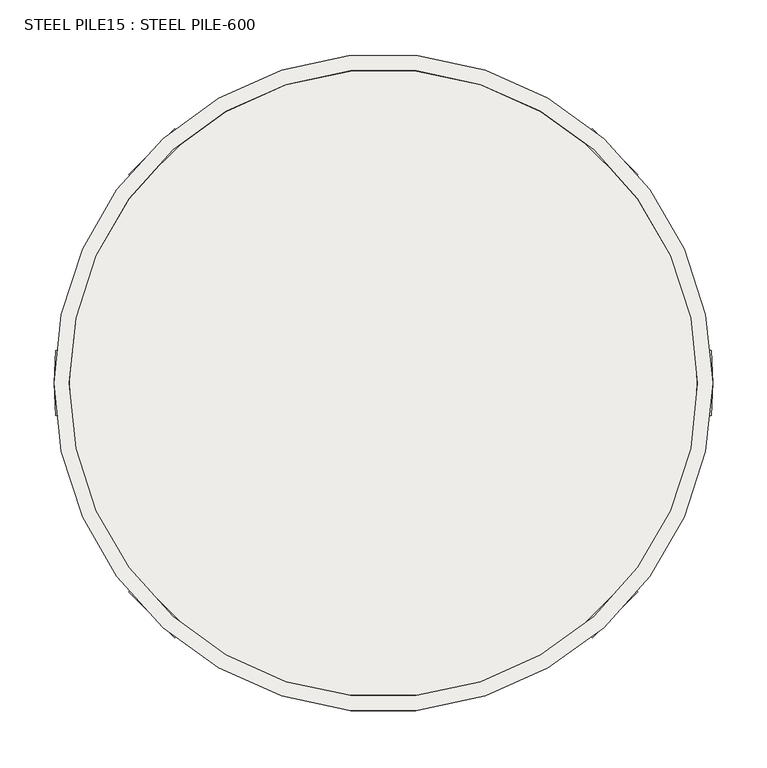
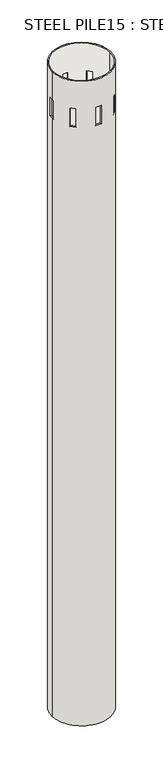
"""IFC4 building model written with IfcOpenShell, lengths in millimetres: slab geometry, STEEL PILE15 : STEEL PILE-600."""

from ifc_helpers import new_model, si_unit, point, frame, frame_2d, origin, place, context, project, spatial, polyline, circle_curve, trimmed, segment, composite_curve, outline, extrude, source, transform, mapped, element, save
from ifc_brep_helpers import plane_surface, cylinder_surface, revolved_surface, advanced_brep


def steel_pile15_steel_pile_600_f495fe2f(model_context):
    return source(origin(), model_context, "Body", "SolidModel", [
        advanced_brep(
        [(7615.5, 66679.5208589, -7500.0), (8224.5, 66679.5208589, -7500.0), (7629.5, 66679.5208589, -7500.0), (8210.5, 66679.5208589, -7500.0), (7615.5, 66679.5208589, -500.0), (8224.5, 66679.5208589, -500.0), (7629.5, 66679.5208589, -500.0), (8210.5, 66679.5208589, -500.0), (8224.5, 66679.5208589, -1000.0), (8223.0185638, 66649.5208589, -1000.0), (8223.0185638, 66649.5208589, -800.0), (8224.5, 66679.5208589, -800.0), (7615.5, 66679.5208589, -800.0), (7616.9814362, 66649.5208589, -800.0), (7616.9814362, 66649.5208589, -1000.0), (7615.5, 66679.5208589, -1000.0), (8155.4796847, 66486.467581, -1000.0), (8113.0532778, 66444.0411742, -1000.0), (8113.0532778, 66444.0411742, -800.0), (8155.4796847, 66486.467581, -800.0), (7950.0, 66376.5022951, -1000.0), (7890.0, 66376.5022951, -1000.0), (7890.0, 66376.5022951, -800.0), (7950.0, 66376.5022951, -800.0), (7726.9467222, 66444.0411742, -1000.0), (7684.5203153, 66486.467581, -1000.0), (7684.5203153, 66486.467581, -800.0), (7726.9467222, 66444.0411742, -800.0), (7616.9814362, 66709.5208589, -1000.0), (7616.9814362, 66709.5208589, -800.0), (8223.0185638, 66709.5208589, -800.0), (8223.0185638, 66709.5208589, -1000.0), (7684.5203153, 66872.5741367, -1000.0), (7726.9467222, 66915.0005436, -1000.0), (7726.9467222, 66915.0005436, -800.0), (7684.5203153, 66872.5741367, -800.0), (7890.0, 66982.5394227, -1000.0), (7950.0, 66982.5394227, -1000.0), (7950.0, 66982.5394227, -800.0), (7890.0, 66982.5394227, -800.0), (8113.0532778, 66915.0005436, -1000.0), (8155.4796847, 66872.5741367, -1000.0), (8155.4796847, 66872.5741367, -800.0), (8113.0532778, 66915.0005436, -800.0), (8210.5, 66679.5208589, -1000.0), (8208.9467944, 66709.5208589, -1000.0), (8208.9467944, 66709.5208589, -800.0), (8210.5, 66679.5208589, -800.0), (7629.5, 66679.5208589, -800.0), (7631.0532056, 66709.5208589, -800.0), (7631.0532056, 66709.5208589, -1000.0), (7629.5, 66679.5208589, -1000.0), (8145.5294412, 66862.6238932, -1000.0), (8103.1030343, 66905.0503001, -1000.0), (8103.1030343, 66905.0503001, -800.0), (8145.5294412, 66862.6238932, -800.0), (7950.0, 66968.4676533, -1000.0), (7890.0, 66968.4676533, -1000.0), (7890.0, 66968.4676533, -800.0), (7950.0, 66968.4676533, -800.0), (7736.8969657, 66905.0503001, -1000.0), (7694.4705588, 66862.6238932, -1000.0), (7694.4705588, 66862.6238932, -800.0), (7736.8969657, 66905.0503001, -800.0), (7631.0532056, 66649.5208589, -1000.0), (7631.0532056, 66649.5208589, -800.0), (8208.9467944, 66649.5208589, -800.0), (8208.9467944, 66649.5208589, -1000.0), (7694.4705588, 66496.4178246, -1000.0), (7736.8969657, 66453.9914177, -1000.0), (7736.8969657, 66453.9914177, -800.0), (7694.4705588, 66496.4178246, -800.0), (7890.0, 66390.5740645, -1000.0), (7950.0, 66390.5740645, -1000.0), (7950.0, 66390.5740645, -800.0), (7890.0, 66390.5740645, -800.0), (8103.1030343, 66453.9914177, -1000.0), (8145.5294412, 66496.4178246, -1000.0), (8145.5294412, 66496.4178246, -800.0), (8103.1030343, 66453.9914177, -800.0)],
        [
            (0, 1, circle_curve(frame((7920.0, 66679.5208589, -7500.0), z_axis=(0.0, 0.0, -1.0), x_axis=(1.0, 0.0, 0.0)), 304.5)),
            (1, 0, circle_curve(frame((7920.0, 66679.5208589, -7500.0), z_axis=(0.0, 0.0, -1.0), x_axis=(1.0, 0.0, 0.0)), 304.5)),
            (2, 3, circle_curve(frame((7920.0, 66679.5208589, -7500.0), z_axis=(0.0, 0.0, 1.0), x_axis=(1.0, 0.0, 0.0)), 290.5)),
            (3, 2, circle_curve(frame((7920.0, 66679.5208589, -7500.0), z_axis=(0.0, 0.0, 1.0), x_axis=(1.0, 0.0, 0.0)), 290.5)),
            (4, 5, circle_curve(frame((7920.0, 66679.5208589, -500.0), z_axis=(0.0, 0.0, 1.0), x_axis=(1.0, 0.0, 0.0)), 304.5)),
            (5, 4, circle_curve(frame((7920.0, 66679.5208589, -500.0), z_axis=(0.0, 0.0, 1.0), x_axis=(1.0, 0.0, 0.0)), 304.5)),
            (6, 7, circle_curve(frame((7920.0, 66679.5208589, -500.0), z_axis=(0.0, 0.0, -1.0), x_axis=(1.0, 0.0, 0.0)), 290.5)),
            (7, 6, circle_curve(frame((7920.0, 66679.5208589, -500.0), z_axis=(0.0, 0.0, -1.0), x_axis=(1.0, 0.0, 0.0)), 290.5)),
            (1, 8),
            (8, 9, circle_curve(frame((7920.0, 66679.5208589, -1000.0), z_axis=(0.0, 0.0, -1.0), x_axis=(1.0, 0.0, 0.0)), 304.5)),
            (9, 10),
            (10, 11, circle_curve(frame((7920.0, 66679.5208589, -800.0), z_axis=(0.0, 0.0, 1.0), x_axis=(1.0, 0.0, 0.0)), 304.5)),
            (11, 5),
            (4, 12),
            (12, 13, circle_curve(frame((7920.0, 66679.5208589, -800.0), z_axis=(0.0, 0.0, 1.0), x_axis=(1.0, 0.0, 0.0)), 304.5)),
            (13, 14),
            (14, 15, circle_curve(frame((7920.0, 66679.5208589, -1000.0), z_axis=(0.0, 0.0, -1.0), x_axis=(1.0, 0.0, 0.0)), 304.5)),
            (15, 0),
            (16, 17, circle_curve(frame((7920.0, 66679.5208589, -1000.0), z_axis=(0.0, 0.0, -1.0), x_axis=(1.0, 0.0, 0.0)), 304.5)),
            (17, 18),
            (18, 19, circle_curve(frame((7920.0, 66679.5208589, -800.0), z_axis=(0.0, 0.0, 1.0), x_axis=(1.0, 0.0, 0.0)), 304.5)),
            (19, 16),
            (20, 21, circle_curve(frame((7920.0, 66679.5208589, -1000.0), z_axis=(0.0, 0.0, -1.0), x_axis=(1.0, 0.0, 0.0)), 304.5)),
            (21, 22),
            (22, 23, circle_curve(frame((7920.0, 66679.5208589, -800.0), z_axis=(0.0, 0.0, 1.0), x_axis=(1.0, 0.0, 0.0)), 304.5)),
            (23, 20),
            (24, 25, circle_curve(frame((7920.0, 66679.5208589, -1000.0), z_axis=(0.0, 0.0, -1.0), x_axis=(1.0, 0.0, 0.0)), 304.5)),
            (25, 26),
            (26, 27, circle_curve(frame((7920.0, 66679.5208589, -800.0), z_axis=(0.0, 0.0, 1.0), x_axis=(1.0, 0.0, 0.0)), 304.5)),
            (27, 24),
            (15, 28, circle_curve(frame((7920.0, 66679.5208589, -1000.0), z_axis=(0.0, 0.0, -1.0), x_axis=(1.0, 0.0, 0.0)), 304.5)),
            (28, 29),
            (29, 12, circle_curve(frame((7920.0, 66679.5208589, -800.0), z_axis=(0.0, 0.0, 1.0), x_axis=(1.0, 0.0, 0.0)), 304.5)),
            (11, 30, circle_curve(frame((7920.0, 66679.5208589, -800.0), z_axis=(0.0, 0.0, 1.0), x_axis=(1.0, 0.0, 0.0)), 304.5)),
            (30, 31),
            (31, 8, circle_curve(frame((7920.0, 66679.5208589, -1000.0), z_axis=(0.0, 0.0, -1.0), x_axis=(1.0, 0.0, 0.0)), 304.5)),
            (32, 33, circle_curve(frame((7920.0, 66679.5208589, -1000.0), z_axis=(0.0, 0.0, -1.0), x_axis=(1.0, 0.0, 0.0)), 304.5)),
            (33, 34),
            (34, 35, circle_curve(frame((7920.0, 66679.5208589, -800.0), z_axis=(0.0, 0.0, 1.0), x_axis=(1.0, 0.0, 0.0)), 304.5)),
            (35, 32),
            (36, 37, circle_curve(frame((7920.0, 66679.5208589, -1000.0), z_axis=(0.0, 0.0, -1.0), x_axis=(1.0, 0.0, 0.0)), 304.5)),
            (37, 38),
            (38, 39, circle_curve(frame((7920.0, 66679.5208589, -800.0), z_axis=(0.0, 0.0, 1.0), x_axis=(1.0, 0.0, 0.0)), 304.5)),
            (39, 36),
            (40, 41, circle_curve(frame((7920.0, 66679.5208589, -1000.0), z_axis=(0.0, 0.0, -1.0), x_axis=(1.0, 0.0, 0.0)), 304.5)),
            (41, 42),
            (42, 43, circle_curve(frame((7920.0, 66679.5208589, -800.0), z_axis=(0.0, 0.0, 1.0), x_axis=(1.0, 0.0, 0.0)), 304.5)),
            (43, 40),
            (3, 44),
            (44, 45, circle_curve(frame((7920.0, 66679.5208589, -1000.0), z_axis=(0.0, 0.0, 1.0), x_axis=(1.0, 0.0, 0.0)), 290.5)),
            (45, 46),
            (46, 47, circle_curve(frame((7920.0, 66679.5208589, -800.0), z_axis=(0.0, 0.0, -1.0), x_axis=(1.0, 0.0, 0.0)), 290.5)),
            (47, 7),
            (6, 48),
            (48, 49, circle_curve(frame((7920.0, 66679.5208589, -800.0), z_axis=(0.0, 0.0, -1.0), x_axis=(1.0, 0.0, 0.0)), 290.5)),
            (49, 50),
            (50, 51, circle_curve(frame((7920.0, 66679.5208589, -1000.0), z_axis=(0.0, 0.0, 1.0), x_axis=(1.0, 0.0, 0.0)), 290.5)),
            (51, 2),
            (52, 53, circle_curve(frame((7920.0, 66679.5208589, -1000.0), z_axis=(0.0, 0.0, 1.0), x_axis=(1.0, 0.0, 0.0)), 290.5)),
            (53, 54),
            (54, 55, circle_curve(frame((7920.0, 66679.5208589, -800.0), z_axis=(0.0, 0.0, -1.0), x_axis=(1.0, 0.0, 0.0)), 290.5)),
            (55, 52),
            (56, 57, circle_curve(frame((7920.0, 66679.5208589, -1000.0), z_axis=(0.0, 0.0, 1.0), x_axis=(1.0, 0.0, 0.0)), 290.5)),
            (57, 58),
            (58, 59, circle_curve(frame((7920.0, 66679.5208589, -800.0), z_axis=(0.0, 0.0, -1.0), x_axis=(1.0, 0.0, 0.0)), 290.5)),
            (59, 56),
            (60, 61, circle_curve(frame((7920.0, 66679.5208589, -1000.0), z_axis=(0.0, 0.0, 1.0), x_axis=(1.0, 0.0, 0.0)), 290.5)),
            (61, 62),
            (62, 63, circle_curve(frame((7920.0, 66679.5208589, -800.0), z_axis=(0.0, 0.0, -1.0), x_axis=(1.0, 0.0, 0.0)), 290.5)),
            (63, 60),
            (51, 64, circle_curve(frame((7920.0, 66679.5208589, -1000.0), z_axis=(0.0, 0.0, 1.0), x_axis=(1.0, 0.0, 0.0)), 290.5)),
            (64, 65),
            (65, 48, circle_curve(frame((7920.0, 66679.5208589, -800.0), z_axis=(0.0, 0.0, -1.0), x_axis=(1.0, 0.0, 0.0)), 290.5)),
            (47, 66, circle_curve(frame((7920.0, 66679.5208589, -800.0), z_axis=(0.0, 0.0, -1.0), x_axis=(1.0, 0.0, 0.0)), 290.5)),
            (66, 67),
            (67, 44, circle_curve(frame((7920.0, 66679.5208589, -1000.0), z_axis=(0.0, 0.0, 1.0), x_axis=(1.0, 0.0, 0.0)), 290.5)),
            (68, 69, circle_curve(frame((7920.0, 66679.5208589, -1000.0), z_axis=(0.0, 0.0, 1.0), x_axis=(1.0, 0.0, 0.0)), 290.5)),
            (69, 70),
            (70, 71, circle_curve(frame((7920.0, 66679.5208589, -800.0), z_axis=(0.0, 0.0, -1.0), x_axis=(1.0, 0.0, 0.0)), 290.5)),
            (71, 68),
            (72, 73, circle_curve(frame((7920.0, 66679.5208589, -1000.0), z_axis=(0.0, 0.0, 1.0), x_axis=(1.0, 0.0, 0.0)), 290.5)),
            (73, 74),
            (74, 75, circle_curve(frame((7920.0, 66679.5208589, -800.0), z_axis=(0.0, 0.0, -1.0), x_axis=(1.0, 0.0, 0.0)), 290.5)),
            (75, 72),
            (76, 77, circle_curve(frame((7920.0, 66679.5208589, -1000.0), z_axis=(0.0, 0.0, 1.0), x_axis=(1.0, 0.0, 0.0)), 290.5)),
            (77, 78),
            (78, 79, circle_curve(frame((7920.0, 66679.5208589, -800.0), z_axis=(0.0, 0.0, -1.0), x_axis=(1.0, 0.0, 0.0)), 290.5)),
            (79, 76),
            (68, 25),
            (24, 69),
            (72, 21),
            (20, 73),
            (76, 17),
            (16, 77),
            (67, 9),
            (31, 45),
            (52, 41),
            (40, 53),
            (56, 37),
            (36, 57),
            (60, 33),
            (32, 61),
            (50, 28),
            (14, 64),
            (13, 65),
            (49, 29),
            (35, 62),
            (63, 34),
            (39, 58),
            (59, 38),
            (43, 54),
            (55, 42),
            (30, 46),
            (66, 10),
            (19, 78),
            (79, 18),
            (23, 74),
            (75, 22),
            (27, 70),
            (71, 26),
        ],
        [
            plane_surface(frame((8224.5, 66679.5208589, -7500.0), z_axis=(0.0, 0.0, -1.0), x_axis=(0.0, -1.0, 0.0))),
            plane_surface(frame((8224.5, 66679.5208589, -500.0), z_axis=(0.0, 0.0, 1.0), x_axis=(0.0, 1.0, 0.0))),
            cylinder_surface(frame((7920.0, 66679.5208589, -7500.0), z_axis=(0.0, 0.0, 1.0), x_axis=(1.0, 0.0, 0.0)), 304.5),
            revolved_surface(polyline([(8210.5, 66679.5208589, -7500.0), (8210.5, 66679.5208589, -500.0)]), (7920.0, 66679.5208589, 200.0), (0.0, 0.0, -1.0)),
            plane_surface(frame((7450.0, 66649.5208589, -1000.0), z_axis=(0.0, 0.0, 1.0), x_axis=(-1.0, 0.0, 0.0))),
            plane_surface(frame((7847.5735931, 66649.5208589, -1000.0), z_axis=(0.0, 1.0, 0.0), x_axis=(0.0, 0.0, 1.0))),
            plane_surface(frame((7450.0, 66709.5208589, -1000.0), z_axis=(0.0, -1.0, 0.0), x_axis=(0.0, 0.0, 1.0))),
            plane_surface(frame((7847.5735931, 66709.5208589, -1000.0), z_axis=(0.7071067811865517, 0.7071067811865435, 0.0), x_axis=(0.0, 0.0, 1.0))),
            plane_surface(frame((7608.8730163, 67033.0742495, -1000.0), z_axis=(-0.7071067811865476, -0.7071067811865476, 0.0), x_axis=(0.0, 0.0, 1.0))),
            plane_surface(frame((7890.0, 66751.9472658, -1000.0), z_axis=(1.0, 0.0, 0.0), x_axis=(0.0, 0.0, 1.0))),
            plane_surface(frame((7950.0, 67149.5208589, -1000.0), z_axis=(-1.0, 0.0, 0.0), x_axis=(0.0, 0.0, 1.0))),
            plane_surface(frame((7950.0, 66751.9472658, -1000.0), z_axis=(0.7071067811865558, -0.7071067811865394, 0.0), x_axis=(0.0, 0.0, 1.0))),
            plane_surface(frame((8273.5533906, 66990.6478426, -1000.0), z_axis=(-0.7071067811865476, 0.7071067811865476, 0.0), x_axis=(0.0, 0.0, 1.0))),
            plane_surface(frame((7992.4264069, 66709.5208589, -1000.0), z_axis=(0.0, -1.0, 0.0), x_axis=(0.0, 0.0, 1.0))),
            plane_surface(frame((8390.0, 66649.5208589, -1000.0), z_axis=(0.0, 1.0, 0.0), x_axis=(0.0, 0.0, 1.0))),
            plane_surface(frame((7992.4264069, 66649.5208589, -1000.0), z_axis=(-0.7071067811865489, -0.7071067811865461, 0.0), x_axis=(0.0, 0.0, 1.0))),
            plane_surface(frame((8231.1269837, 66325.9674683, -1000.0), z_axis=(0.7071067811865517, 0.7071067811865435, 0.0), x_axis=(0.0, 0.0, 1.0))),
            plane_surface(frame((7950.0, 66607.094452, -1000.0), z_axis=(-1.0, 0.0, 0.0), x_axis=(0.0, 0.0, 1.0))),
            plane_surface(frame((7890.0, 66209.5208589, -1000.0), z_axis=(1.0, 0.0, 0.0), x_axis=(0.0, 0.0, 1.0))),
            plane_surface(frame((7890.0, 66607.094452, -1000.0), z_axis=(-0.7071067811865448, 0.7071067811865502, 0.0), x_axis=(0.0, 0.0, 1.0))),
            plane_surface(frame((7566.4466094, 66368.3938752, -1000.0), z_axis=(0.7071067811865489, -0.7071067811865461, 0.0), x_axis=(0.0, 0.0, 1.0))),
            plane_surface(frame((7450.0, 66649.5208589, -800.0), z_axis=(0.0, 0.0, -1.0), x_axis=(1.0, 0.0, 0.0))),
        ],
        [
            (0, [[1, 2], [3, 4]]),
            (1, [[5, 6], [7, 8]]),
            (2, [[-2, 9, 10, 11, 12, 13, -5, 14, 15, 16, 17, 18], [19, 20, 21, 22], [23, 24, 25, 26], [27, 28, 29, 30]]),
            (2, [[-1, -18, 31, 32, 33, -14, -6, -13, 34, 35, 36, -9], [37, 38, 39, 40], [41, 42, 43, 44], [45, 46, 47, 48]]),
            (3, [[-4, 49, 50, 51, 52, 53, -7, 54, 55, 56, 57, 58], [59, 60, 61, 62], [63, 64, 65, 66], [67, 68, 69, 70]]),
            (3, [[-3, -58, 71, 72, 73, -54, -8, -53, 74, 75, 76, -49], [77, 78, 79, 80], [81, 82, 83, 84], [85, 86, 87, 88]]),
            (4, [[89, -27, 90, -77]]),
            (4, [[91, -23, 92, -81]]),
            (4, [[93, -19, 94, -85]]),
            (4, [[95, -10, -36, 96, -50, -76]]),
            (4, [[97, -45, 98, -59]]),
            (4, [[99, -41, 100, -63]]),
            (4, [[101, -37, 102, -67]]),
            (4, [[103, -31, -17, 104, -71, -57]]),
            (5, [[-104, -16, 105, -72]]),
            (6, [[-103, -56, 106, -32]]),
            (7, [[-102, -40, 107, -68]]),
            (8, [[-101, -70, 108, -38]]),
            (9, [[-100, -44, 109, -64]]),
            (10, [[-99, -66, 110, -42]]),
            (11, [[-98, -48, 111, -60]]),
            (12, [[-97, -62, 112, -46]]),
            (13, [[-96, -35, 113, -51]]),
            (14, [[-95, -75, 114, -11]]),
            (15, [[-94, -22, 115, -86]]),
            (16, [[-93, -88, 116, -20]]),
            (17, [[-92, -26, 117, -82]]),
            (18, [[-91, -84, 118, -24]]),
            (19, [[-90, -30, 119, -78]]),
            (20, [[-89, -80, 120, -28]]),
            (21, [[-107, -39, -108, -69]]),
            (21, [[-109, -43, -110, -65]]),
            (21, [[-111, -47, -112, -61]]),
            (21, [[-113, -34, -12, -114, -74, -52]]),
            (21, [[-105, -15, -33, -106, -55, -73]]),
            (21, [[-115, -21, -116, -87]]),
            (21, [[-117, -25, -118, -83]]),
            (21, [[-119, -29, -120, -79]]),
        ],
    ),
        extrude(outline(composite_curve([segment(trimmed(circle_curve(frame_2d((7920.0, 66679.5208589)), 290.5), [point((7629.5, 66679.5208589))], [point((8210.5, 66679.5208589))], False, "CARTESIAN"), True, "CONTINUOUS"), segment(trimmed(circle_curve(frame_2d((7920.0, 66679.5208589)), 290.5), [point((8210.5, 66679.5208589))], [point((7629.5, 66679.5208589))], False, "CARTESIAN"), True, "CONTINUOUS")], self_intersect=False)), frame((0.0, 0.0, -2530.0), z_axis=(0.0, 0.0, 1.0), x_axis=(1.0, 0.0, 0.0)), (0.0, 0.0, 1.0), 30.0),
    ])


if __name__ == "__main__":
    model = new_model("IFC4")
    model_context = context("Model", 3, world=origin())
    ifc_project = project(units=[si_unit("LENGTHUNIT", "METRE", prefix="MILLI")], contexts=[model_context])
    site = spatial("IfcSite", under=ifc_project)
    building = spatial("IfcBuilding", under=site)
    placement = place(None, origin())
    steel_pile15_steel_pile_600_shape = steel_pile15_steel_pile_600_f495fe2f(model_context)
    element("IfcSlab", 1, ObjectType="STEEL PILE15 : STEEL PILE-600", at=placement, inside=building, context=model_context, shape_type="MappedRepresentation", body=[
        mapped(steel_pile15_steel_pile_600_shape, transform((0.0, 0.0, 0.0), x_axis=(1.0, 0.0, 0.0), y_axis=(0.0, 1.0, 0.0), z_axis=(0.0, 0.0, 1.0))),
    ])
    save(model, "model.ifc")

# Revit data of these elements
# Element 1 (IfcSlab, "STEEL PILE15 : STEEL PILE-600")
#   Materials on its faces: "Metal - Steel"
# Materials
#   "Metal - Steel": class "Metal", colour RGB 247 247 247, transparency 0, Cost = 0
